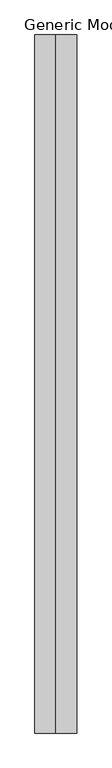
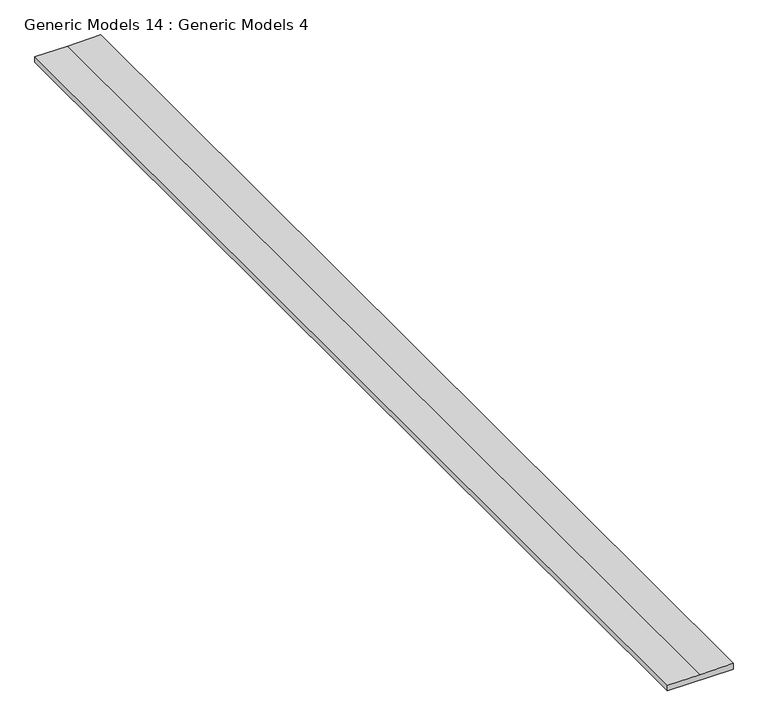
"""IFC4 building model written with IfcOpenShell, lengths in millimetres: proxy geometry, Generic Models 14 : Generic Models 4."""

from ifc_helpers import new_model, si_unit, frame, origin, place, context, project, spatial, polyline, outline, extrude, source, transform, mapped, element, save


def generic_models_14_generic_models_4_af54af74(model_context):
    return source(origin(), model_context, "Body", "SweptSolid", [
        extrude(outline(polyline([(126790.196, 7276.9263704), (126790.196, 8394.5263704), (126894.7036609, 8394.5263704), (126883.0619942, 7835.7263704), (126894.7036609, 7276.9263704), (126790.196, 7276.9263704)])), frame((0.0, -6864.9230338, 0.0), z_axis=(0.0, 1.0, 0.0), x_axis=(0.0, 0.0, 1.0)), (0.0, 0.0, 1.0), 18643.6),
    ])


if __name__ == "__main__":
    model = new_model("IFC4")
    model_context = context("Model", 3, world=origin())
    ifc_project = project(units=[si_unit("LENGTHUNIT", "METRE", prefix="MILLI")], contexts=[model_context])
    site = spatial("IfcSite", under=ifc_project)
    building = spatial("IfcBuilding", under=site)
    placement = place(None, origin())
    generic_models_14_generic_models_4_shape = generic_models_14_generic_models_4_af54af74(model_context)
    element("IfcBuildingElementProxy", 1, Name="Generic Models 14 : Generic Models 4", ObjectType="Generic Models 14 : Generic Models 4", at=placement, inside=building, context=model_context, shape_type="MappedRepresentation", body=[
        mapped(generic_models_14_generic_models_4_shape, transform((0.0, 0.0, 0.0), x_axis=(1.0, 0.0, 0.0), y_axis=(0.0, 1.0, 0.0), z_axis=(0.0, 0.0, 1.0))),
    ])
    save(model, "model.ifc")

# Revit data of these elements
# Element 1 (IfcBuildingElementProxy, "Generic Models 14 : Generic Models 4")
#   Materials on its faces: "_TAPERED 2X BLOCKING (1% SLOPE) - SLOPED TOWARD DRAINS (SEE ROOF PLAN)"
# Materials
#   "_TAPERED 2X BLOCKING (1% SLOPE) - SLOPED TOWARD DRAINS (SEE ROOF PLAN)": class "Generic", colour RGB 177 130 114, transparency 0, Cost = 0
